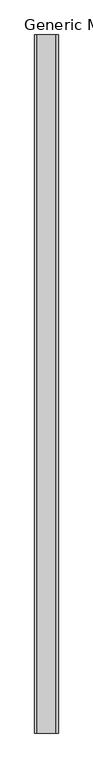
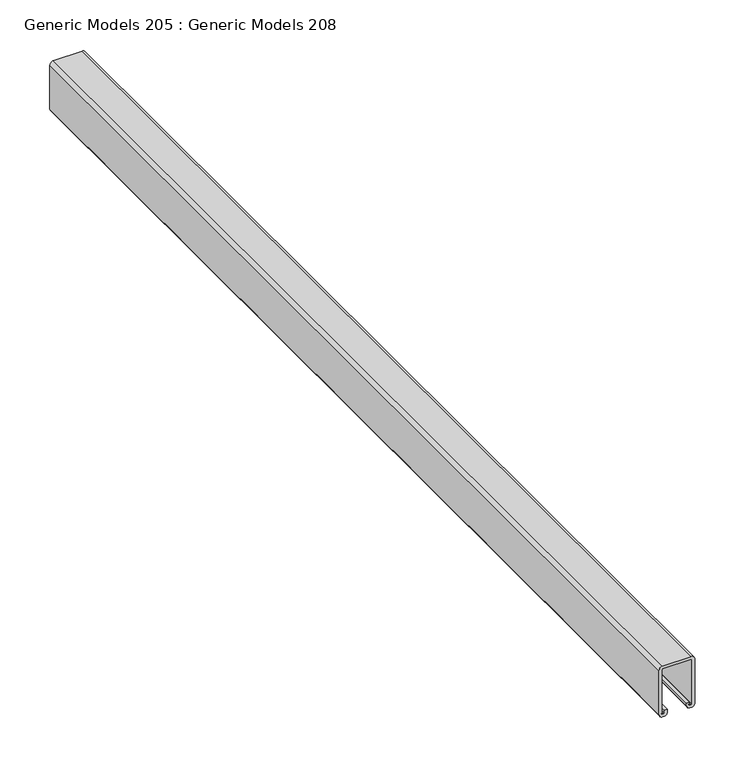
"""IFC4 building model written with IfcOpenShell, lengths in millimetres: proxy geometry, Generic Models 205 : Generic Models 208."""

from ifc_helpers import new_model, si_unit, point, frame, frame_2d, origin, place, context, project, spatial, polyline, circle_curve, trimmed, segment, composite_curve, outline, extrude, source, transform, mapped, element, save


def generic_models_205_generic_models_208_e10493e2(model_context):
    return source(origin(), model_context, "Body", "SweptSolid", [
        extrude(outline(composite_curve([segment(polyline([(2071.434878, 53673.981697), (2074.6253412, 53673.981697), (2074.6253412, 53670.806697), (2071.434878, 53670.806697)]), True, "CONTINUOUS"), segment(trimmed(circle_curve(frame_2d((2071.434878, 53670.0284102)), 0.7782868), [point((2071.434878, 53670.806697))], [point((2070.6565912, 53670.0284102))], True, "CARTESIAN"), True, "CONTINUOUS"), segment(polyline([(2070.6565912, 53670.0284102), (2070.6565912, 53668.4821558)]), True, "CONTINUOUS"), segment(trimmed(circle_curve(frame_2d((2071.50705, 53668.4821558)), 0.8504588), [point((2070.6565912, 53668.4821558))], [point((2071.50705, 53667.631697))], True, "CARTESIAN"), True, "CONTINUOUS"), segment(polyline([(2071.50705, 53667.631697), (2125.3702466, 53667.631697)]), True, "CONTINUOUS"), segment(trimmed(circle_curve(frame_2d((2125.3702466, 53668.4805416)), 0.8488446), [point((2125.3702466, 53667.631697))], [point((2126.2190912, 53668.4805416))], True, "CARTESIAN"), True, "CONTINUOUS"), segment(polyline([(2126.2190912, 53668.4805416), (2126.2190912, 53701.7473741)]), True, "CONTINUOUS"), segment(trimmed(circle_curve(frame_2d((2125.4097683, 53701.7473741)), 0.8093229), [point((2126.2190912, 53701.7473741))], [point((2125.4097683, 53702.556697))], True, "CARTESIAN"), True, "CONTINUOUS"), segment(polyline([(2125.4097683, 53702.556697), (2071.4935001, 53702.556697)]), True, "CONTINUOUS"), segment(trimmed(circle_curve(frame_2d((2071.4935001, 53701.7197881)), 0.8369089), [point((2071.4935001, 53702.556697))], [point((2070.6565912, 53701.7197881))], True, "CARTESIAN"), True, "CONTINUOUS"), segment(polyline([(2070.6565912, 53701.7197881), (2070.6565912, 53700.2509999)]), True, "CONTINUOUS"), segment(trimmed(circle_curve(frame_2d((2071.5258942, 53700.2509999)), 0.8693029), [point((2070.6565912, 53700.2509999))], [point((2071.5258942, 53699.381697))], True, "CARTESIAN"), True, "CONTINUOUS"), segment(polyline([(2071.5258942, 53699.381697), (2074.6253412, 53699.381697), (2074.6253412, 53696.206697), (2071.5258942, 53696.206697)]), True, "CONTINUOUS"), segment(trimmed(circle_curve(frame_2d((2071.5258942, 53700.2509999)), 4.0443029), [point((2071.5258942, 53696.206697))], [point((2067.4815912, 53700.2509999))], False, "CARTESIAN"), True, "CONTINUOUS"), segment(polyline([(2067.4815912, 53700.2509999), (2067.4815912, 53701.7197881)]), True, "CONTINUOUS"), segment(trimmed(circle_curve(frame_2d((2071.4935001, 53701.7197881)), 4.0119089), [point((2067.4815912, 53701.7197881))], [point((2071.4935001, 53705.731697))], False, "CARTESIAN"), True, "CONTINUOUS"), segment(polyline([(2071.4935001, 53705.731697), (2125.4097683, 53705.731697)]), True, "CONTINUOUS"), segment(trimmed(circle_curve(frame_2d((2125.4097683, 53701.7473741)), 3.9843229), [point((2125.4097683, 53705.731697))], [point((2129.3940912, 53701.7473741))], False, "CARTESIAN"), True, "CONTINUOUS"), segment(polyline([(2129.3940912, 53701.7473741), (2129.3940912, 53668.4805416)]), True, "CONTINUOUS"), segment(trimmed(circle_curve(frame_2d((2125.3702466, 53668.4805416)), 4.0238446), [point((2129.3940912, 53668.4805416))], [point((2125.3702466, 53664.456697))], False, "CARTESIAN"), True, "CONTINUOUS"), segment(polyline([(2125.3702466, 53664.456697), (2071.50705, 53664.456697)]), True, "CONTINUOUS"), segment(trimmed(circle_curve(frame_2d((2071.50705, 53668.4821558)), 4.0254588), [point((2071.50705, 53664.456697))], [point((2067.4815912, 53668.4821558))], False, "CARTESIAN"), True, "CONTINUOUS"), segment(polyline([(2067.4815912, 53668.4821558), (2067.4815912, 53670.0284102)]), True, "CONTINUOUS"), segment(trimmed(circle_curve(frame_2d((2071.434878, 53670.0284102)), 3.9532868), [point((2067.4815912, 53670.0284102))], [point((2071.434878, 53673.981697))], False, "CARTESIAN"), True, "CONTINUOUS")], self_intersect=False)), frame((0.0, -228.7033818, 0.0), z_axis=(0.0, 1.0, 0.0), x_axis=(0.0, 0.0, 1.0)), (0.0, 0.0, 1.0), 1219.2),
    ])


if __name__ == "__main__":
    model = new_model("IFC4")
    model_context = context("Model", 3, world=origin())
    ifc_project = project(units=[si_unit("LENGTHUNIT", "METRE", prefix="MILLI")], contexts=[model_context])
    site = spatial("IfcSite", under=ifc_project)
    building = spatial("IfcBuilding", under=site)
    placement = place(None, origin())
    generic_models_205_generic_models_208_shape = generic_models_205_generic_models_208_e10493e2(model_context)
    element("IfcBuildingElementProxy", 1, Name="Generic Models 205 : Generic Models 208", ObjectType="Generic Models 205 : Generic Models 208", at=placement, inside=building, context=model_context, shape_type="MappedRepresentation", body=[
        mapped(generic_models_205_generic_models_208_shape, transform((0.0, 0.0, 0.0), x_axis=(1.0, 0.0, 0.0), y_axis=(0.0, 1.0, 0.0), z_axis=(0.0, 0.0, 1.0))),
    ])
    save(model, "model.ifc")

# Revit data of these elements
# Element 1 (IfcBuildingElementProxy, "Generic Models 205 : Generic Models 208")
#   Materials on its faces: "GALVANIZED UNISTRUT P5500, 1 5/8\" X 2 7/16\" OR ALUM. CHANNEL"
# Materials
#   "GALVANIZED UNISTRUT P5500, 1 5/8\" X 2 7/16\" OR ALUM. CHANNEL": class "Metal", colour RGB 244 244 244, transparency 0, Description = "Aluminum 6061", Cost = 0
